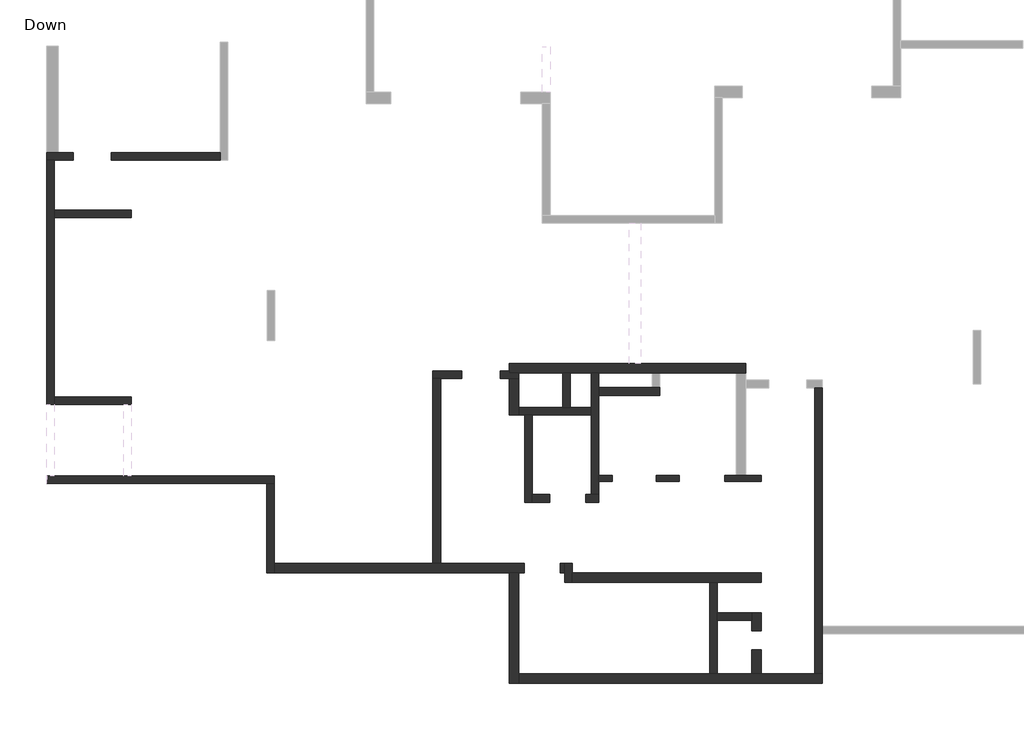
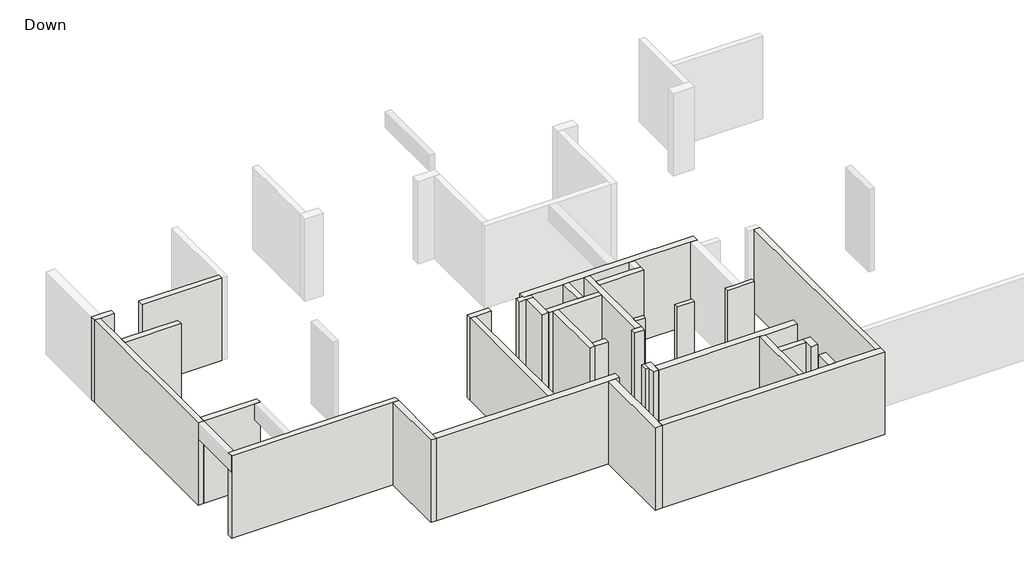
# One storey, part 1 of 2: 33 walls.
"""IFC4 building model written with IfcOpenShell, lengths in millimetres."""

from ifc_helpers import new_model, si_unit, origin, origin_with_axes, place, context, project, spatial, polyline, outline, extrude, faceted_brep, element, save

model = new_model("IFC4")

# Units and contexts
model_context = context("Model", 3, world=origin())
ifc_project = project(units=[si_unit("LENGTHUNIT", "METRE", prefix="MILLI")], contexts=[model_context])

# Site, building, storey
site = spatial("IfcSite", under=ifc_project)
building = spatial("IfcBuilding", under=site)
storey = spatial("IfcBuildingStorey", under=building, Name="Down", Elevation=0.0)

# Walls
placement = place(None, origin())
element("IfcWall", 1, ObjectType="15", at=placement, inside=storey, context=model_context, shape_type="Brep", body=[
    faceted_brep([(-5557.7212244, 6644.9881336, 0.0), (-5957.7212244, 6644.9881336, 0.0), (-6207.7212244, 6644.9881336, 0.0), (-6502.9843823, 6644.9881336, 0.0), (-6502.9843823, 6644.9881336, 3100.0), (-6207.7212244, 6644.9881336, 3100.0), (-5957.7212244, 6644.9881336, 3100.0), (-5557.7212244, 6644.9881336, 3100.0), (-5557.7212244, 6644.9881336, 2920.0), (-5557.7212244, 6494.9881336, 0.0), (-5557.7212244, 6494.9881336, 2920.0), (-5557.7212244, 6494.9881336, 3100.0), (-6502.9843823, 6494.9881336, 3100.0), (-6502.9843823, 6494.9881336, 2920.0), (-6502.9843823, 6494.9881336, 0.0), (-6502.9843823, 6644.4618178, 3100.0)], [[[0, 1, 2, 3, 4, 5, 6, 7, 8]], [[9, 10, 11, 12, 13, 14]], [[3, 2, 1, 0, 9, 14]], [[4, 3, 14, 13, 12, 15]], [[7, 6, 5, 4, 15, 12, 11]], [[0, 8, 7, 11, 10, 9]]]),
])
element("IfcWall", 2, ObjectType="15", at=placement, inside=storey, context=model_context, shape_type="Brep", body=[
    faceted_brep([(-7696.6685928, 6644.4618178, 0.0), (-8294.5633296, 6644.4618178, 0.0), (-8294.5633296, 6644.4618178, 2920.0), (-8294.5633296, 6644.4618178, 3100.0), (-7696.6685928, 6644.4618178, 3100.0), (-7696.6685928, 6644.4618178, 2920.0), (-7696.6685928, 6494.4618178, 0.0), (-7696.6685928, 6494.4618178, 2920.0), (-7696.6685928, 6494.4618178, 3100.0), (-8294.5633296, 6494.4618178, 3100.0), (-8294.5633296, 6494.4618178, 2920.0), (-8294.5633296, 6494.4618178, 0.0)], [[[0, 1, 2, 3, 4, 5]], [[6, 7, 8, 9, 10, 11]], [[1, 0, 6, 11]], [[3, 2, 1, 11, 10, 9]], [[4, 3, 9, 8]], [[0, 5, 4, 8, 7, 6]]]),
])
element("IfcWall", 3, ObjectType="15", at=placement, inside=storey, context=model_context, shape_type="Brep", body=[
    faceted_brep([(-9437.7212244, 6644.4618178, 0.0), (-9785.0896454, 6644.4618178, 0.0), (-9785.0896454, 6644.4618178, 3100.0), (-9437.7212244, 6644.4618178, 3100.0), (-9437.7212244, 6644.4618178, 2920.0), (-9437.7212244, 6494.4618178, 0.0), (-9437.7212244, 6494.4618178, 2920.0), (-9437.7212244, 6494.4618178, 3100.0), (-9785.0896454, 6494.4618178, 3100.0), (-9785.0896454, 6494.4618178, 2920.0), (-9785.0896454, 6494.4618178, 0.0)], [[[0, 1, 2, 3, 4]], [[5, 6, 7, 8, 9, 10]], [[1, 0, 5, 10]], [[3, 2, 8, 7]], [[0, 4, 3, 7, 6, 5]], [[2, 1, 10, 9, 8]]]),
])
element("IfcWall", 4, ObjectType="20", at=placement, inside=storey, context=model_context, shape_type="Brep", body=[
    faceted_brep([(-19660.8791191, 15061.303923, 0.0), (-22490.8791191, 15061.303923, 0.0), (-22490.8791191, 15061.303923, 2920.0), (-22490.8791191, 15061.303923, 3100.0), (-19660.8791191, 15061.303923, 3100.0), (-19660.8791191, 15061.303923, 2920.0), (-19660.8791191, 14861.303923, 0.0), (-19660.8791191, 14861.303923, 3100.0), (-22490.8791191, 14861.303923, 3100.0), (-22490.8791191, 14861.303923, 2920.0), (-22490.8791191, 14861.303923, 0.0)], [[[0, 1, 2, 3, 4, 5]], [[6, 7, 8, 9, 10]], [[1, 0, 6, 10]], [[3, 2, 1, 10, 9, 8]], [[4, 3, 8, 7]], [[0, 5, 4, 7, 6]]]),
])
element("IfcWall", 5, ObjectType="20", at=placement, inside=storey, context=model_context, shape_type="Brep", body=[
    faceted_brep([(-23484.0370138, 15061.303923, 0.0), (-23878.7738559, 15061.303923, 0.0), (-24178.7738559, 15061.303923, 0.0), (-24180.8791191, 15061.303923, 0.0), (-24180.8791191, 15061.303923, 3100.0), (-24178.7738559, 15061.303923, 3100.0), (-23878.7738559, 15061.303923, 3100.0), (-23484.0370138, 15061.303923, 3100.0), (-23484.0370138, 15061.303923, 2920.0), (-23484.0370138, 14861.303923, 0.0), (-23484.0370138, 14861.303923, 2920.0), (-23484.0370138, 14861.303923, 3100.0), (-23980.8791191, 14861.303923, 3100.0), (-24180.8791191, 14861.303923, 3100.0), (-24180.8791191, 14861.303923, 0.0), (-23980.8791191, 14861.303923, 0.0)], [[[0, 1, 2, 3, 4, 5, 6, 7, 8]], [[9, 10, 11, 12, 13, 14, 15]], [[3, 2, 1, 0, 9, 15, 14]], [[7, 6, 5, 4, 13, 12, 11]], [[0, 8, 7, 11, 10, 9]], [[4, 3, 14, 13]]]),
])
element("IfcWall", 6, ObjectType="20", at=placement, inside=storey, context=model_context, shape_type="Brep", body=[
    faceted_brep([(-24180.8791191, 14861.303923, 0.0), (-24180.8791191, 8497.0933967, 0.0), (-24180.8791191, 8497.0933967, 2500.0), (-24180.8791191, 8497.0933967, 3100.0), (-24180.8791191, 14861.303923, 3100.0), (-23980.8791191, 14861.303923, 0.0), (-23980.8791191, 14861.303923, 2920.0), (-23980.8791191, 14861.303923, 3100.0), (-23980.8791191, 13568.6723441, 3100.0), (-23980.8791191, 13368.6723441, 3100.0), (-23980.8791191, 8697.0933967, 3100.0), (-23980.8791191, 8497.0933967, 3100.0), (-23980.8791191, 8497.0933967, 2500.0), (-23980.8791191, 8497.0933967, 0.0), (-23980.8791191, 8697.0933967, 0.0), (-23980.8791191, 13368.6723441, 0.0), (-23980.8791191, 13568.6723441, 0.0)], [[[0, 1, 2, 3, 4]], [[5, 6, 7, 8, 9, 10, 11, 12, 13, 14, 15, 16]], [[1, 0, 5, 16, 15, 14, 13]], [[4, 3, 11, 10, 9, 8, 7]], [[0, 4, 7, 6, 5]], [[3, 2, 1, 13, 12, 11]]]),
])
element("IfcWall", 7, ObjectType="20", at=placement, inside=storey, context=model_context, shape_type="Brep", body=[
    faceted_brep([(-23980.8791191, 13368.6723441, 0.0), (-21970.3528033, 13368.6723441, 0.0), (-21970.3528033, 13368.6723441, 2920.0), (-21970.3528033, 13368.6723441, 3100.0), (-23980.8791191, 13368.6723441, 3100.0), (-23980.8791191, 13368.6723441, 2920.0), (-23980.8791191, 13568.6723441, 0.0), (-23980.8791191, 13568.6723441, 2920.0), (-23980.8791191, 13568.6723441, 3100.0), (-21970.3528033, 13568.6723441, 3100.0), (-21970.3528033, 13568.6723441, 2920.0), (-21970.3528033, 13568.6723441, 0.0)], [[[0, 1, 2, 3, 4, 5]], [[6, 7, 8, 9, 10, 11]], [[1, 0, 6, 11]], [[3, 2, 1, 11, 10, 9]], [[4, 3, 9, 8]], [[0, 5, 4, 8, 7, 6]]]),
])
element("IfcWall", 8, ObjectType="20", at=placement, inside=storey, context=model_context, shape_type="Brep", body=[
    faceted_brep([(-23980.8791191, 8497.0933967, 0.0), (-21970.3528033, 8497.0933967, 0.0), (-21970.3528033, 8497.0933967, 3100.0), (-22170.3528033, 8497.0933967, 3100.0), (-23980.8791191, 8497.0933967, 3100.0), (-23980.8791191, 8497.0933967, 2920.0), (-23980.8791191, 8697.0933967, 0.0), (-23980.8791191, 8697.0933967, 2920.0), (-23980.8791191, 8697.0933967, 3100.0), (-21970.3528033, 8697.0933967, 3100.0), (-21970.3528033, 8697.0933967, 2920.0), (-21970.3528033, 8697.0933967, 0.0)], [[[0, 1, 2, 3, 4, 5]], [[6, 7, 8, 9, 10, 11]], [[1, 0, 6, 11]], [[2, 1, 11, 10, 9]], [[4, 3, 2, 9, 8]], [[0, 5, 4, 8, 7, 6]]]),
])
element("IfcWall", 9, ObjectType="20", at=placement, inside=storey, context=model_context, shape_type="Brep", body=[
    faceted_brep([(-24178.7738559, 6438.1460283, 0.0), (-18441.9317507, 6438.1460283, 0.0), (-18241.9317507, 6438.1460283, 0.0), (-18241.9317507, 6438.1460283, 3100.0), (-18441.9317507, 6438.1460283, 3100.0), (-24178.7738559, 6438.1460283, 3100.0), (-24178.7738559, 6638.1460283, 0.0), (-24178.7738559, 6638.1460283, 3100.0), (-23980.8791191, 6638.1460283, 3100.0), (-22170.3528033, 6638.1460283, 3100.0), (-21970.3528033, 6638.1460283, 3100.0), (-18241.9317507, 6638.1460283, 3100.0), (-18241.9317507, 6638.1460283, 2920.0), (-18241.9317507, 6638.1460283, 0.0)], [[[0, 1, 2, 3, 4, 5]], [[6, 7, 8, 9, 10, 11, 12, 13]], [[2, 1, 0, 6, 13]], [[5, 4, 3, 11, 10, 9, 8, 7]], [[0, 5, 7, 6]], [[3, 2, 13, 12, 11]]]),
])
element("IfcWall", 10, ObjectType="20", at=placement, inside=storey, context=model_context, shape_type="Brep", body=[
    faceted_brep([(-18441.9317507, 6438.1460283, 0.0), (-18441.9317507, 4107.6197125, 0.0), (-18441.9317507, 4107.6197125, 3100.0), (-18441.9317507, 6438.1460283, 3100.0), (-18241.9317507, 6438.1460283, 0.0), (-18241.9317507, 6438.1460283, 3100.0), (-18241.9317507, 4357.6197125, 3100.0), (-18241.9317507, 4107.6197125, 3100.0), (-18241.9317507, 4107.6197125, 0.0), (-18241.9317507, 4357.6197125, 0.0)], [[[0, 1, 2, 3]], [[4, 5, 6, 7, 8, 9]], [[1, 0, 4, 9, 8]], [[3, 2, 7, 6, 5]], [[0, 3, 5, 4]], [[2, 1, 8, 7]]]),
])
element("IfcWall", 11, ObjectType="20", at=placement, inside=storey, context=model_context, shape_type="SweptSolid", body=[
    extrude(outline(polyline([(-6700.8791191, 3063.4091862), (-5809.8264875, 3063.4091862), (-5809.8264875, 2863.4091862), (-6700.8791191, 2863.4091862), (-6700.8791191, 3063.4091862)])), origin_with_axes(), (0.0, 0.0, 1.0), 3100.0),
])
element("IfcWall", 12, ObjectType="20", at=placement, inside=storey, context=model_context, shape_type="Brep", body=[
    faceted_brep([(-6700.8791191, 1473.4091862, 0.0), (-6700.8791191, 2863.4091862, 0.0), (-6700.8791191, 3063.4091862, 0.0), (-6700.8791191, 3859.1986599, 0.0), (-6700.8791191, 3859.1986599, 3100.0), (-6700.8791191, 3063.4091862, 3100.0), (-6700.8791191, 2863.4091862, 3100.0), (-6700.8791191, 1473.4091862, 3100.0), (-6900.8791191, 1473.4091862, 0.0), (-6900.8791191, 1473.4091862, 3100.0), (-6900.8791191, 3859.1986599, 3100.0), (-6900.8791191, 3859.1986599, 0.0)], [[[0, 1, 2, 3, 4, 5, 6, 7]], [[8, 9, 10, 11]], [[3, 2, 1, 0, 8, 11]], [[7, 6, 5, 4, 10, 9]], [[4, 3, 11, 10]], [[0, 7, 9, 8]]]),
])
element("IfcWall", 13, ObjectType="20", at=placement, inside=storey, context=model_context, shape_type="Brep", body=[
    faceted_brep([(-10481.9317507, 3859.1986599, 0.0), (-10481.9317507, 4109.1986599, 0.0), (-10481.9317507, 4358.1460283, 0.0), (-10481.9317507, 4358.1460283, 2920.0), (-10481.9317507, 4358.1460283, 3100.0), (-10481.9317507, 4109.1986599, 3100.0), (-10481.9317507, 3859.1986599, 3100.0), (-10681.9317507, 3859.1986599, 0.0), (-10681.9317507, 3859.1986599, 2920.0), (-10681.9317507, 3859.1986599, 3100.0), (-10681.9317507, 4108.1460283, 3100.0), (-10681.9317507, 4358.1460283, 3100.0), (-10681.9317507, 4358.1460283, 0.0), (-10681.9317507, 4108.1460283, 0.0)], [[[0, 1, 2, 3, 4, 5, 6]], [[7, 8, 9, 10, 11, 12, 13]], [[2, 1, 0, 7, 13, 12]], [[6, 5, 4, 11, 10, 9]], [[0, 6, 9, 8, 7]], [[4, 3, 2, 12, 11]]]),
])
element("IfcWall", 14, ObjectType="20", at=placement, inside=storey, context=model_context, shape_type="Brep", body=[
    faceted_brep([(-3966.142277, 1473.4091862, 0.0), (-3966.142277, 2516.0407652, 0.0), (-3966.142277, 2716.0407652, 0.0), (-3966.142277, 8930.7776073, 0.0), (-3966.142277, 8930.7776073, 3100.0), (-3966.142277, 2716.0407652, 3100.0), (-3966.142277, 2516.0407652, 3100.0), (-3966.142277, 1473.4091862, 3100.0), (-4166.142277, 1473.4091862, 0.0), (-4166.142277, 1473.4091862, 2920.0), (-4166.142277, 1473.4091862, 3100.0), (-4166.142277, 8930.7776073, 3100.0), (-4166.142277, 8930.7776073, 2920.0), (-4166.142277, 8930.7776073, 0.0)], [[[0, 1, 2, 3, 4, 5, 6, 7]], [[8, 9, 10, 11, 12, 13]], [[3, 2, 1, 0, 8, 13]], [[7, 6, 5, 4, 11, 10]], [[4, 3, 13, 12, 11]], [[0, 7, 10, 9, 8]]]),
])
element("IfcWall", 15, ObjectType="20", at=placement, inside=storey, context=model_context, shape_type="Brep", body=[
    faceted_brep([(-9785.0896454, 6147.6197125, 0.0), (-9785.0896454, 6494.4618178, 0.0), (-9785.0896454, 6644.4618178, 0.0), (-9785.0896454, 8732.8828704, 0.0), (-9785.0896454, 8932.8828704, 0.0), (-9785.0896454, 9312.3565546, 0.0), (-9785.0896454, 9312.3565546, 3100.0), (-9785.0896454, 8932.8828704, 3100.0), (-9785.0896454, 8732.8828704, 3100.0), (-9785.0896454, 6644.4618178, 3100.0), (-9785.0896454, 6494.4618178, 3100.0), (-9785.0896454, 6147.6197125, 3100.0), (-9985.0896454, 6147.6197125, 0.0), (-9985.0896454, 6147.6197125, 2920.0), (-9985.0896454, 6147.6197125, 3100.0), (-9985.0896454, 8219.1986599, 3100.0), (-9985.0896454, 8419.1986599, 3100.0), (-9985.0896454, 9312.3565546, 3100.0), (-9985.0896454, 9312.3565546, 0.0), (-9985.0896454, 8419.1986599, 0.0), (-9985.0896454, 8219.1986599, 0.0)], [[[0, 1, 2, 3, 4, 5, 6, 7, 8, 9, 10, 11]], [[12, 13, 14, 15, 16, 17, 18, 19, 20]], [[5, 4, 3, 2, 1, 0, 12, 20, 19, 18]], [[11, 10, 9, 8, 7, 6, 17, 16, 15, 14]], [[6, 5, 18, 17]], [[0, 11, 14, 13, 12]]]),
])
element("IfcWall", 16, ObjectType="20", at=placement, inside=storey, context=model_context, shape_type="SweptSolid", body=[
    extrude(outline(polyline([(-10728.2475402, 8419.1986599), (-10728.2475402, 9312.3565546), (-10528.2475402, 9312.3565546), (-10528.2475402, 8419.1986599), (-10728.2475402, 8419.1986599)])), origin_with_axes(), (0.0, 0.0, 1.0), 3100.0),
])
element("IfcWall", 17, ObjectType="20", at=placement, inside=storey, context=model_context, shape_type="Brep", body=[
    faceted_brep([(-9785.0896454, 8732.8828704, 0.0), (-8195.6159612, 8732.8828704, 0.0), (-8195.6159612, 8732.8828704, 3100.0), (-9785.0896454, 8732.8828704, 3100.0), (-9785.0896454, 8932.8828704, 0.0), (-9785.0896454, 8932.8828704, 3100.0), (-8395.6159612, 8932.8828704, 3100.0), (-8195.6159612, 8932.8828704, 3100.0), (-8195.6159612, 8932.8828704, 0.0), (-8395.6159612, 8932.8828704, 0.0)], [[[0, 1, 2, 3]], [[4, 5, 6, 7, 8, 9]], [[1, 0, 4, 9, 8]], [[3, 2, 7, 6, 5]], [[0, 3, 5, 4]], [[2, 1, 8, 7]]]),
])
element("IfcWall", 18, ObjectType="20", at=placement, inside=storey, context=model_context, shape_type="Brep", body=[
    faceted_brep([(-11874.0370138, 8219.1986599, 0.0), (-11726.142277, 8219.1986599, 0.0), (-11526.142277, 8219.1986599, 0.0), (-9985.0896454, 8219.1986599, 0.0), (-9985.0896454, 8219.1986599, 2920.0), (-9985.0896454, 8219.1986599, 3100.0), (-11526.142277, 8219.1986599, 3100.0), (-11726.142277, 8219.1986599, 3100.0), (-11874.0370138, 8219.1986599, 3100.0), (-11874.0370138, 8419.1986599, 0.0), (-11874.0370138, 8419.1986599, 3100.0), (-10728.2475402, 8419.1986599, 3100.0), (-10528.2475402, 8419.1986599, 3100.0), (-9985.0896454, 8419.1986599, 3100.0), (-9985.0896454, 8419.1986599, 0.0), (-10528.2475402, 8419.1986599, 0.0), (-10728.2475402, 8419.1986599, 0.0)], [[[0, 1, 2, 3, 4, 5, 6, 7, 8]], [[9, 10, 11, 12, 13, 14, 15, 16]], [[3, 2, 1, 0, 9, 16, 15, 14]], [[8, 7, 6, 5, 13, 12, 11, 10]], [[0, 8, 10, 9]], [[5, 4, 3, 14, 13]]]),
])
element("IfcWall", 19, ObjectType="20", at=placement, inside=storey, context=model_context, shape_type="Brep", body=[
    faceted_brep([(-11726.142277, 8219.1986599, 0.0), (-11726.142277, 5947.6197125, 0.0), (-11726.142277, 5947.6197125, 2920.0), (-11726.142277, 5947.6197125, 3100.0), (-11726.142277, 8219.1986599, 3100.0), (-11726.142277, 8219.1986599, 2920.0), (-11526.142277, 8219.1986599, 0.0), (-11526.142277, 8219.1986599, 2920.0), (-11526.142277, 8219.1986599, 3100.0), (-11526.142277, 6147.6197125, 3100.0), (-11526.142277, 5947.6197125, 3100.0), (-11526.142277, 5947.6197125, 0.0), (-11526.142277, 6147.6197125, 0.0)], [[[0, 1, 2, 3, 4, 5]], [[6, 7, 8, 9, 10, 11, 12]], [[1, 0, 6, 12, 11]], [[4, 3, 10, 9, 8]], [[0, 5, 4, 8, 7, 6]], [[3, 2, 1, 11, 10]]]),
])
element("IfcWall", 20, ObjectType="20", at=placement, inside=storey, context=model_context, shape_type="Brep", body=[
    faceted_brep([(-11526.142277, 5947.6197125, 0.0), (-11069.3001717, 5947.6197125, 0.0), (-11069.3001717, 5947.6197125, 2920.0), (-11069.3001717, 5947.6197125, 3100.0), (-11526.142277, 5947.6197125, 3100.0), (-11526.142277, 6147.6197125, 0.0), (-11526.142277, 6147.6197125, 2920.0), (-11526.142277, 6147.6197125, 3100.0), (-11069.3001717, 6147.6197125, 3100.0), (-11069.3001717, 6147.6197125, 2920.0), (-11069.3001717, 6147.6197125, 0.0)], [[[0, 1, 2, 3, 4]], [[5, 6, 7, 8, 9, 10]], [[1, 0, 5, 10]], [[3, 2, 1, 10, 9, 8]], [[4, 3, 8, 7]], [[0, 4, 7, 6, 5]]]),
])
element("IfcWall", 21, ObjectType="20", at=placement, inside=storey, context=model_context, shape_type="Brep", body=[
    faceted_brep([(-10124.0370138, 5947.6197125, 0.0), (-9785.0896454, 5947.6197125, 0.0), (-9785.0896454, 5947.6197125, 2920.0), (-9785.0896454, 5947.6197125, 3100.0), (-10124.0370138, 5947.6197125, 3100.0), (-10124.0370138, 5947.6197125, 2920.0), (-10124.0370138, 6147.6197125, 0.0), (-10124.0370138, 6147.6197125, 2920.0), (-10124.0370138, 6147.6197125, 3100.0), (-9985.0896454, 6147.6197125, 3100.0), (-9785.0896454, 6147.6197125, 3100.0), (-9785.0896454, 6147.6197125, 0.0), (-9985.0896454, 6147.6197125, 0.0)], [[[0, 1, 2, 3, 4, 5]], [[6, 7, 8, 9, 10, 11, 12]], [[1, 0, 6, 12, 11]], [[4, 3, 10, 9, 8]], [[0, 5, 4, 8, 7, 6]], [[3, 2, 1, 11, 10]]]),
])
element("IfcWall", 22, ObjectType="20", at=placement, inside=storey, context=model_context, shape_type="Brep", body=[
    faceted_brep([(-12364.0370138, 9370.9220034, 0.0), (-12364.0370138, 9370.9220034, 2920.0), (-12364.0370138, 9370.9220034, 3100.0), (-12124.0370138, 9370.9220034, 3100.0), (-12124.0370138, 9370.9220034, 2920.0), (-12124.0370138, 9370.9220034, 0.0), (-12364.0370138, 9170.9220034, 0.0), (-12124.0370138, 9170.9220034, 0.0), (-11874.0370138, 9170.9220034, 0.0), (-11874.0370138, 9170.9220034, 3100.0), (-12124.0370138, 9170.9220034, 3100.0), (-12364.0370138, 9170.9220034, 3100.0), (-12364.0370138, 9170.9220034, 2920.0), (-12124.0370138, 9312.3565546, 0.0), (-11874.0370138, 9312.3565546, 0.0), (-11874.0370138, 9312.3565546, 3100.0), (-12124.0370138, 9312.3565546, 3100.0)], [[[0, 1, 2, 3, 4, 5]], [[6, 7, 8, 9, 10, 11, 12]], [[8, 7, 6, 0, 5, 13, 14]], [[2, 1, 0, 6, 12, 11]], [[11, 10, 9, 15, 16, 3, 2]], [[9, 8, 14, 15]], [[13, 16, 15, 14]], [[16, 13, 5, 4, 3]]]),
])
element("IfcWall", 23, ObjectType="20", at=placement, inside=storey, context=model_context, shape_type="Brep", body=[
    faceted_brep([(-13360.7601979, 9370.9220034, 0.0), (-14113.5106981, 9370.9220034, 0.0), (-14113.5106981, 9370.9220034, 2920.0), (-14113.5106981, 9370.9220034, 3100.0), (-13360.7601979, 9370.9220034, 3100.0), (-13360.7601979, 9370.9220034, 2920.0), (-13360.7601979, 9170.9220034, 0.0), (-13360.7601979, 9170.9220034, 2920.0), (-13360.7601979, 9170.9220034, 3100.0), (-13913.5106981, 9170.9220034, 3100.0), (-14113.5106981, 9170.9220034, 3100.0), (-14113.5106981, 9170.9220034, 0.0), (-13913.5106981, 9170.9220034, 0.0)], [[[0, 1, 2, 3, 4, 5]], [[6, 7, 8, 9, 10, 11, 12]], [[1, 0, 6, 12, 11]], [[4, 3, 10, 9, 8]], [[0, 5, 4, 8, 7, 6]], [[3, 2, 1, 11, 10]]]),
])
element("IfcWall", 24, ObjectType="20", at=placement, inside=storey, context=model_context, shape_type="Brep", body=[
    faceted_brep([(-14113.5106981, 9170.9220034, 0.0), (-14113.5106981, 4357.6197125, 0.0), (-14113.5106981, 4357.6197125, 2920.0), (-14113.5106981, 4357.6197125, 3100.0), (-14113.5106981, 9170.9220034, 3100.0), (-13913.5106981, 9170.9220034, 0.0), (-13913.5106981, 9170.9220034, 2920.0), (-13913.5106981, 9170.9220034, 3100.0), (-13913.5106981, 4357.6197125, 3100.0), (-13913.5106981, 4357.6197125, 2920.0), (-13913.5106981, 4357.6197125, 0.0)], [[[0, 1, 2, 3, 4]], [[5, 6, 7, 8, 9, 10]], [[1, 0, 5, 10]], [[4, 3, 8, 7]], [[0, 4, 7, 6, 5]], [[3, 2, 1, 10, 9, 8]]]),
])
element("IfcWall", 25, ObjectType="25", at=placement, inside=storey, context=model_context, shape_type="Brep", body=[
    faceted_brep([(-18241.9317507, 4107.6197125, 0.0), (-12125.6159612, 4107.6197125, 0.0), (-11875.6159612, 4107.6197125, 0.0), (-11736.6685928, 4107.6197125, 0.0), (-11736.6685928, 4107.6197125, 2920.0), (-11736.6685928, 4107.6197125, 3100.0), (-11875.6159612, 4107.6197125, 3100.0), (-12125.6159612, 4107.6197125, 3100.0), (-18241.9317507, 4107.6197125, 3100.0), (-18241.9317507, 4357.6197125, 0.0), (-18241.9317507, 4357.6197125, 2920.0), (-18241.9317507, 4357.6197125, 3100.0), (-14113.5106981, 4357.6197125, 3100.0), (-13913.5106981, 4357.6197125, 3100.0), (-11736.6685928, 4357.6197125, 3100.0), (-11736.6685928, 4357.6197125, 2920.0), (-11736.6685928, 4357.6197125, 0.0), (-13913.5106981, 4357.6197125, 0.0), (-14113.5106981, 4357.6197125, 0.0)], [[[0, 1, 2, 3, 4, 5, 6, 7, 8]], [[9, 10, 11, 12, 13, 14, 15, 16, 17, 18]], [[3, 2, 1, 0, 9, 18, 17, 16]], [[5, 4, 3, 16, 15, 14]], [[8, 7, 6, 5, 14, 13, 12, 11]], [[0, 8, 11, 10, 9]]]),
])
element("IfcWall", 26, ObjectType="25", at=placement, inside=storey, context=model_context, shape_type="Brep", body=[
    faceted_brep([(-12125.6159612, 4107.6197125, 0.0), (-12125.6159612, 1223.4091862, 0.0), (-12125.6159612, 1223.4091862, 3100.0), (-12125.6159612, 4107.6197125, 3100.0), (-11875.6159612, 4107.6197125, 0.0), (-11875.6159612, 4107.6197125, 2920.0), (-11875.6159612, 4107.6197125, 3100.0), (-11875.6159612, 1473.4091862, 3100.0), (-11875.6159612, 1223.4091862, 3100.0), (-11875.6159612, 1223.4091862, 0.0), (-11875.6159612, 1473.4091862, 0.0)], [[[0, 1, 2, 3]], [[4, 5, 6, 7, 8, 9, 10]], [[1, 0, 4, 10, 9]], [[3, 2, 8, 7, 6]], [[0, 3, 6, 5, 4]], [[2, 1, 9, 8]]]),
])
element("IfcWall", 27, ObjectType="25", at=placement, inside=storey, context=model_context, shape_type="Brep", body=[
    faceted_brep([(-11875.6159612, 1223.4091862, 0.0), (-3966.142277, 1223.4091862, 0.0), (-3966.142277, 1223.4091862, 3100.0), (-11875.6159612, 1223.4091862, 3100.0), (-11875.6159612, 1473.4091862, 0.0), (-11875.6159612, 1473.4091862, 2920.0), (-11875.6159612, 1473.4091862, 3100.0), (-10462.9843823, 1473.4091862, 3100.0), (-6900.8791191, 1473.4091862, 3100.0), (-6700.8791191, 1473.4091862, 3100.0), (-5809.8264875, 1473.4091862, 3100.0), (-5559.8264875, 1473.4091862, 3100.0), (-4166.142277, 1473.4091862, 3100.0), (-3966.142277, 1473.4091862, 3100.0), (-3966.142277, 1473.4091862, 0.0), (-4166.142277, 1473.4091862, 0.0), (-5559.8264875, 1473.4091862, 0.0), (-5809.8264875, 1473.4091862, 0.0), (-6700.8791191, 1473.4091862, 0.0), (-6900.8791191, 1473.4091862, 0.0)], [[[0, 1, 2, 3]], [[4, 5, 6, 7, 8, 9, 10, 11, 12, 13, 14, 15, 16, 17, 18, 19]], [[1, 0, 4, 19, 18, 17, 16, 15, 14]], [[3, 2, 13, 12, 11, 10, 9, 8, 7, 6]], [[0, 3, 6, 5, 4]], [[2, 1, 14, 13]]]),
])
element("IfcWall", 28, ObjectType="25", at=placement, inside=storey, context=model_context, shape_type="Brep", body=[
    faceted_brep([(-5559.8264875, 1473.4091862, 0.0), (-5559.8264875, 2094.9881336, 0.0), (-5559.8264875, 2094.9881336, 3100.0), (-5559.8264875, 1473.4091862, 3100.0), (-5559.8264875, 1473.4091862, 2920.0), (-5809.8264875, 1473.4091862, 0.0), (-5809.8264875, 1473.4091862, 3100.0), (-5809.8264875, 2094.9881336, 3100.0), (-5809.8264875, 2094.9881336, 0.0)], [[[0, 1, 2, 3, 4]], [[5, 6, 7, 8]], [[1, 0, 5, 8]], [[2, 1, 8, 7]], [[3, 2, 7, 6]], [[0, 4, 3, 6, 5]]]),
])
element("IfcWall", 29, ObjectType="25", at=placement, inside=storey, context=model_context, shape_type="Brep", body=[
    faceted_brep([(-5559.8264875, 2591.8302388, 0.0), (-5559.8264875, 3063.4091862, 0.0), (-5559.8264875, 3063.4091862, 3100.0), (-5559.8264875, 2591.8302388, 3100.0), (-5809.8264875, 2591.8302388, 0.0), (-5809.8264875, 2591.8302388, 3100.0), (-5809.8264875, 2863.4091862, 3100.0), (-5809.8264875, 3063.4091862, 3100.0), (-5809.8264875, 3063.4091862, 0.0), (-5809.8264875, 2863.4091862, 0.0)], [[[0, 1, 2, 3]], [[4, 5, 6, 7, 8, 9]], [[1, 0, 4, 9, 8]], [[3, 2, 7, 6, 5]], [[0, 3, 5, 4]], [[2, 1, 8, 7]]]),
])
element("IfcWall", 30, ObjectType="25", at=placement, inside=storey, context=model_context, shape_type="Brep", body=[
    faceted_brep([(-5559.8264875, 4109.1986599, 0.0), (-10481.9317507, 4109.1986599, 0.0), (-10481.9317507, 4109.1986599, 2920.0), (-10481.9317507, 4109.1986599, 3100.0), (-5559.8264875, 4109.1986599, 3100.0), (-5559.8264875, 4109.1986599, 2920.0), (-5559.8264875, 3859.1986599, 0.0), (-5559.8264875, 3859.1986599, 3100.0), (-6700.8791191, 3859.1986599, 3100.0), (-6900.8791191, 3859.1986599, 3100.0), (-10462.9843823, 3859.1986599, 3100.0), (-10481.9317507, 3859.1986599, 3100.0), (-10481.9317507, 3859.1986599, 0.0), (-6900.8791191, 3859.1986599, 0.0), (-6700.8791191, 3859.1986599, 0.0)], [[[0, 1, 2, 3, 4, 5]], [[6, 7, 8, 9, 10, 11, 12, 13, 14]], [[1, 0, 6, 14, 13, 12]], [[4, 3, 11, 10, 9, 8, 7]], [[0, 5, 4, 7, 6]], [[3, 2, 1, 12, 11]]]),
])
element("IfcWall", 31, ObjectType="25", at=placement, inside=storey, context=model_context, shape_type="Brep", body=[
    faceted_brep([(-10681.9317507, 4358.1460283, 0.0), (-10791.4054349, 4358.1460283, 0.0), (-10791.4054349, 4358.1460283, 2920.0), (-10791.4054349, 4358.1460283, 3100.0), (-10681.9317507, 4358.1460283, 3100.0), (-10681.9317507, 4108.1460283, 0.0), (-10681.9317507, 4108.1460283, 2920.0), (-10681.9317507, 4108.1460283, 3100.0), (-10791.4054349, 4108.1460283, 3100.0), (-10791.4054349, 4108.1460283, 2920.0), (-10791.4054349, 4108.1460283, 0.0)], [[[0, 1, 2, 3, 4]], [[5, 6, 7, 8, 9, 10]], [[1, 0, 5, 10]], [[3, 2, 1, 10, 9, 8]], [[4, 3, 8, 7]], [[0, 4, 7, 6, 5]]]),
])
element("IfcWall", 32, ObjectType="25", at=placement, inside=storey, context=model_context, shape_type="Brep", body=[
    faceted_brep([(-5957.7212244, 9562.3565546, 0.0), (-12124.0370138, 9562.3565546, 0.0), (-12124.0370138, 9562.3565546, 2920.0), (-12124.0370138, 9562.3565546, 3100.0), (-8991.4054349, 9562.3565546, 3100.0), (-8691.4054349, 9562.3565546, 3100.0), (-5957.7212244, 9562.3565546, 3100.0), (-5957.7212244, 9562.3565546, 2920.0), (-5957.7212244, 9312.3565546, 0.0), (-5957.7212244, 9312.3565546, 3100.0), (-6207.7212244, 9312.3565546, 3100.0), (-8195.6159612, 9312.3565546, 3100.0), (-8395.6159612, 9312.3565546, 3100.0), (-9785.0896454, 9312.3565546, 3100.0), (-9985.0896454, 9312.3565546, 3100.0), (-10528.2475402, 9312.3565546, 3100.0), (-10728.2475402, 9312.3565546, 3100.0), (-11874.0370138, 9312.3565546, 3100.0), (-12124.0370138, 9312.3565546, 3100.0), (-12124.0370138, 9312.3565546, 0.0), (-11874.0370138, 9312.3565546, 0.0), (-10728.2475402, 9312.3565546, 0.0), (-10528.2475402, 9312.3565546, 0.0), (-9985.0896454, 9312.3565546, 0.0), (-9785.0896454, 9312.3565546, 0.0), (-8395.6159612, 9312.3565546, 0.0), (-8195.6159612, 9312.3565546, 0.0), (-6207.7212244, 9312.3565546, 0.0), (-12124.0370138, 9370.9220034, 0.0), (-12124.0370138, 9370.9220034, 3100.0)], [[[0, 1, 2, 3, 4, 5, 6, 7]], [[8, 9, 10, 11, 12, 13, 14, 15, 16, 17, 18, 19, 20, 21, 22, 23, 24, 25, 26, 27]], [[1, 0, 8, 27, 26, 25, 24, 23, 22, 21, 20, 19, 28]], [[3, 2, 1, 28, 19, 18, 29]], [[6, 5, 4, 3, 29, 18, 17, 16, 15, 14, 13, 12, 11, 10, 9]], [[0, 7, 6, 9, 8]]]),
])
element("IfcWall", 33, ObjectType="25", at=placement, inside=storey, context=model_context, shape_type="Brep", body=[
    faceted_brep([(-12124.0370138, 9170.9220034, 0.0), (-12124.0370138, 8219.1986599, 0.0), (-12124.0370138, 8219.1986599, 2920.0), (-12124.0370138, 8219.1986599, 3100.0), (-12124.0370138, 9170.9220034, 3100.0), (-12124.0370138, 9170.9220034, 2920.0), (-11874.0370138, 9170.9220034, 0.0), (-11874.0370138, 9170.9220034, 3100.0), (-11874.0370138, 8419.1986599, 3100.0), (-11874.0370138, 8219.1986599, 3100.0), (-11874.0370138, 8219.1986599, 0.0), (-11874.0370138, 8419.1986599, 0.0)], [[[0, 1, 2, 3, 4, 5]], [[6, 7, 8, 9, 10, 11]], [[1, 0, 6, 11, 10]], [[4, 3, 9, 8, 7]], [[3, 2, 1, 10, 9]], [[0, 5, 4, 7, 6]]]),
])

save(model, "model.ifc")

# Revit data of these elements
# Project information
#   Project Issue Date = "Issue Date"
#   Project Status = "Project Status"
#   Client Name = "לקוח"
#   Project Address = "Enter address here"
#   Project Name = "Project 037"
#   Project Number = "מספר פרויקט"
# Type "15"
#   Layers, outside or top first: 15 cm "Concrete" (function 1)
# Type "20"
#   Layers, outside or top first: 20 cm "Concrete" (function 1)
# Type "25"
#   Layers, outside or top first: 25 cm "Concrete" (function 1)
# Element 1 (IfcWall, "15")
#   Comments = ""
#   Mark = "W61"
#   SOFiSTiK_EdgeZones = "W69"
#   SOFiSTiK_AMG_Comments = ""
#   Top Offset = 0 cm
#   Base Offset = 0 cm
#   wall height = 310 cm
#   SOFiSTiK_AMG_Scheduled = yes
#   SOFiSTiK_AMG_Adjusted = yes
#   Phase Created = New Construction
#   Base Constraint = Down
#   Top Constraint = Typical Floor
#   Materials on its faces: "Concrete"
# Element 2 (IfcWall, "15")
#   Comments = ""
#   Mark = "W62"
#   SOFiSTiK_EdgeZones = "W70"
#   SOFiSTiK_AMG_Comments = ""
#   Top Offset = 0 cm
#   Base Offset = 0 cm
#   wall height = 310 cm
#   SOFiSTiK_AMG_Scheduled = yes
#   SOFiSTiK_AMG_Adjusted = yes
#   Phase Created = New Construction
#   Base Constraint = Down
#   Top Constraint = Typical Floor
#   Materials on its faces: "Concrete"
# Element 3 (IfcWall, "15")
#   Comments = ""
#   Mark = "W63"
#   SOFiSTiK_EdgeZones = "W71"
#   SOFiSTiK_AMG_Comments = ""
#   Top Offset = 0 cm
#   Base Offset = 0 cm
#   wall height = 310 cm
#   SOFiSTiK_AMG_Scheduled = yes
#   SOFiSTiK_AMG_Adjusted = yes
#   Phase Created = New Construction
#   Base Constraint = Down
#   Top Constraint = Typical Floor
#   Materials on its faces: "Concrete"
# Element 4 (IfcWall, "20")
#   Comments = ""
#   Mark = "W3"
#   SOFiSTiK_EdgeZones = "W3"
#   SOFiSTiK_AMG_Comments = ""
#   Top Offset = 0 cm
#   Base Offset = 0 cm
#   wall height = 310 cm
#   SOFiSTiK_AMG_Scheduled = yes
#   SOFiSTiK_AMG_Adjusted = yes
#   Phase Created = New Construction
#   Base Constraint = Down
#   Top Constraint = Typical Floor
#   Materials on its faces: "Concrete"
# Element 5 (IfcWall, "20")
#   Comments = ""
#   Mark = "W4"
#   SOFiSTiK_EdgeZones = "W4"
#   SOFiSTiK_AMG_Comments = ""
#   Top Offset = 0 cm
#   Base Offset = 0 cm
#   wall height = 310 cm
#   SOFiSTiK_AMG_Scheduled = yes
#   SOFiSTiK_AMG_Adjusted = yes
#   Phase Created = New Construction
#   Base Constraint = Down
#   Top Constraint = Typical Floor
#   Materials on its faces: "Concrete"
# Element 6 (IfcWall, "20")
#   Comments = ""
#   Mark = "W5"
#   SOFiSTiK_EdgeZones = "W5"
#   SOFiSTiK_AMG_Comments = ""
#   Top Offset = 0 cm
#   Base Offset = 0 cm
#   wall height = 310 cm
#   SOFiSTiK_AMG_Scheduled = yes
#   SOFiSTiK_AMG_Adjusted = yes
#   Phase Created = New Construction
#   Base Constraint = Down
#   Top Constraint = Typical Floor
#   Materials on its faces: "Concrete"
# Element 7 (IfcWall, "20")
#   Comments = ""
#   Mark = "W6"
#   SOFiSTiK_EdgeZones = "W6"
#   SOFiSTiK_AMG_Comments = ""
#   Top Offset = 0 cm
#   Base Offset = 0 cm
#   wall height = 310 cm
#   SOFiSTiK_AMG_Scheduled = yes
#   SOFiSTiK_AMG_Adjusted = yes
#   Phase Created = New Construction
#   Base Constraint = Down
#   Top Constraint = Typical Floor
#   Materials on its faces: "Concrete"
# Element 8 (IfcWall, "20")
#   Comments = ""
#   Mark = "W7"
#   SOFiSTiK_EdgeZones = "W7"
#   SOFiSTiK_AMG_Comments = ""
#   Top Offset = 0 cm
#   Base Offset = 0 cm
#   wall height = 310 cm
#   SOFiSTiK_AMG_Scheduled = yes
#   SOFiSTiK_AMG_Adjusted = yes
#   Phase Created = New Construction
#   Base Constraint = Down
#   Top Constraint = Typical Floor
#   Materials on its faces: "Concrete"
# Element 9 (IfcWall, "20")
#   Comments = ""
#   Mark = "W8"
#   SOFiSTiK_EdgeZones = "W8"
#   SOFiSTiK_AMG_Comments = ""
#   Top Offset = 0 cm
#   Base Offset = 0 cm
#   wall height = 310 cm
#   SOFiSTiK_AMG_Scheduled = yes
#   SOFiSTiK_AMG_Adjusted = yes
#   Phase Created = New Construction
#   Base Constraint = Down
#   Top Constraint = Typical Floor
#   Materials on its faces: "Concrete"
# Element 10 (IfcWall, "20")
#   Comments = ""
#   Mark = "W9"
#   SOFiSTiK_EdgeZones = "W9"
#   SOFiSTiK_AMG_Comments = ""
#   Top Offset = 0 cm
#   Base Offset = 0 cm
#   wall height = 310 cm
#   SOFiSTiK_AMG_Scheduled = yes
#   SOFiSTiK_AMG_Adjusted = yes
#   Phase Created = New Construction
#   Base Constraint = Down
#   Top Constraint = Typical Floor
#   Materials on its faces: "Concrete"
# Element 11 (IfcWall, "20")
#   Comments = ""
#   Mark = "W10"
#   SOFiSTiK_EdgeZones = "W10"
#   SOFiSTiK_AMG_Comments = ""
#   Top Offset = 0 cm
#   Base Offset = 0 cm
#   wall height = 310 cm
#   SOFiSTiK_AMG_Scheduled = yes
#   SOFiSTiK_AMG_Adjusted = yes
#   Phase Created = New Construction
#   Base Constraint = Down
#   Top Constraint = Typical Floor
#   Materials on its faces: "Concrete"
# Element 12 (IfcWall, "20")
#   Comments = ""
#   Mark = "W11"
#   SOFiSTiK_EdgeZones = "W12"
#   SOFiSTiK_AMG_Comments = ""
#   Top Offset = 0 cm
#   Base Offset = 0 cm
#   wall height = 310 cm
#   SOFiSTiK_AMG_Scheduled = yes
#   SOFiSTiK_AMG_Adjusted = yes
#   Phase Created = New Construction
#   Base Constraint = Down
#   Top Constraint = Typical Floor
#   Materials on its faces: "Concrete"
# Element 13 (IfcWall, "20")
#   Comments = ""
#   Mark = "W12"
#   SOFiSTiK_EdgeZones = "W13"
#   SOFiSTiK_AMG_Comments = ""
#   Top Offset = 0 cm
#   Base Offset = 0 cm
#   wall height = 310 cm
#   SOFiSTiK_AMG_Scheduled = yes
#   SOFiSTiK_AMG_Adjusted = yes
#   Phase Created = New Construction
#   Base Constraint = Down
#   Top Constraint = Typical Floor
#   Materials on its faces: "Concrete"
# Element 14 (IfcWall, "20")
#   Comments = ""
#   Mark = "W29"
#   SOFiSTiK_EdgeZones = "W34"
#   SOFiSTiK_AMG_Comments = ""
#   Top Offset = 0 cm
#   Base Offset = 0 cm
#   wall height = 310 cm
#   SOFiSTiK_AMG_Scheduled = yes
#   SOFiSTiK_AMG_Adjusted = yes
#   Phase Created = New Construction
#   Base Constraint = Down
#   Top Constraint = Typical Floor
#   Materials on its faces: "Concrete"
# Element 15 (IfcWall, "20")
#   Comments = ""
#   Mark = "W32"
#   SOFiSTiK_EdgeZones = "W37"
#   SOFiSTiK_AMG_Comments = ""
#   Top Offset = 0 cm
#   Base Offset = 0 cm
#   wall height = 310 cm
#   SOFiSTiK_AMG_Scheduled = yes
#   SOFiSTiK_AMG_Adjusted = yes
#   Phase Created = New Construction
#   Base Constraint = Down
#   Top Constraint = Typical Floor
#   Materials on its faces: "Concrete"
# Element 16 (IfcWall, "20")
#   Comments = ""
#   Mark = "W33"
#   SOFiSTiK_EdgeZones = "W38"
#   SOFiSTiK_AMG_Comments = ""
#   Top Offset = 0 cm
#   Base Offset = 0 cm
#   wall height = 310 cm
#   SOFiSTiK_AMG_Scheduled = yes
#   SOFiSTiK_AMG_Adjusted = yes
#   Phase Created = New Construction
#   Base Constraint = Down
#   Top Constraint = Typical Floor
#   Materials on its faces: "Concrete"
# Element 17 (IfcWall, "20")
#   Comments = ""
#   Mark = "W34"
#   SOFiSTiK_EdgeZones = "W39"
#   SOFiSTiK_AMG_Comments = ""
#   Top Offset = 0 cm
#   Base Offset = 0 cm
#   wall height = 310 cm
#   SOFiSTiK_AMG_Scheduled = yes
#   SOFiSTiK_AMG_Adjusted = yes
#   Phase Created = New Construction
#   Base Constraint = Down
#   Top Constraint = Typical Floor
#   Materials on its faces: "Concrete"
# Element 18 (IfcWall, "20")
#   Comments = ""
#   Mark = "W36"
#   SOFiSTiK_EdgeZones = "W41"
#   SOFiSTiK_AMG_Comments = ""
#   Top Offset = 0 cm
#   Base Offset = 0 cm
#   wall height = 310 cm
#   SOFiSTiK_AMG_Scheduled = yes
#   SOFiSTiK_AMG_Adjusted = yes
#   Phase Created = New Construction
#   Base Constraint = Down
#   Top Constraint = Typical Floor
#   Materials on its faces: "Concrete"
# Element 19 (IfcWall, "20")
#   Comments = ""
#   Mark = "W37"
#   SOFiSTiK_EdgeZones = "W42"
#   SOFiSTiK_AMG_Comments = ""
#   Top Offset = 0 cm
#   Base Offset = 0 cm
#   wall height = 310 cm
#   SOFiSTiK_AMG_Scheduled = yes
#   SOFiSTiK_AMG_Adjusted = yes
#   Phase Created = New Construction
#   Base Constraint = Down
#   Top Constraint = Typical Floor
#   Materials on its faces: "Concrete"
# Element 20 (IfcWall, "20")
#   Comments = ""
#   Mark = "W38"
#   SOFiSTiK_EdgeZones = "W43"
#   SOFiSTiK_AMG_Comments = ""
#   Top Offset = 0 cm
#   Base Offset = 0 cm
#   wall height = 310 cm
#   SOFiSTiK_AMG_Scheduled = yes
#   SOFiSTiK_AMG_Adjusted = yes
#   Phase Created = New Construction
#   Base Constraint = Down
#   Top Constraint = Typical Floor
#   Materials on its faces: "Concrete"
# Element 21 (IfcWall, "20")
#   Comments = ""
#   Mark = "W39"
#   SOFiSTiK_EdgeZones = "W44"
#   SOFiSTiK_AMG_Comments = ""
#   Top Offset = 0 cm
#   Base Offset = 0 cm
#   wall height = 310 cm
#   SOFiSTiK_AMG_Scheduled = yes
#   SOFiSTiK_AMG_Adjusted = yes
#   Phase Created = New Construction
#   Base Constraint = Down
#   Top Constraint = Typical Floor
#   Materials on its faces: "Concrete"
# Element 22 (IfcWall, "20")
#   Comments = ""
#   Mark = "W40"
#   SOFiSTiK_EdgeZones = "W46"
#   SOFiSTiK_AMG_Comments = ""
#   Top Offset = 0 cm
#   Base Offset = 0 cm
#   wall height = 310 cm
#   SOFiSTiK_AMG_Scheduled = yes
#   SOFiSTiK_AMG_Adjusted = yes
#   Phase Created = New Construction
#   Base Constraint = Down
#   Top Constraint = Typical Floor
#   Materials on its faces: "Concrete"
# Element 23 (IfcWall, "20")
#   Comments = ""
#   Mark = "W41"
#   SOFiSTiK_EdgeZones = "W47"
#   SOFiSTiK_AMG_Comments = ""
#   Top Offset = 0 cm
#   Base Offset = 0 cm
#   wall height = 310 cm
#   SOFiSTiK_AMG_Scheduled = yes
#   SOFiSTiK_AMG_Adjusted = yes
#   Phase Created = New Construction
#   Base Constraint = Down
#   Top Constraint = Typical Floor
#   Materials on its faces: "Concrete"
# Element 24 (IfcWall, "20")
#   Comments = ""
#   Mark = "W42"
#   SOFiSTiK_EdgeZones = "W48"
#   SOFiSTiK_AMG_Comments = ""
#   Top Offset = 0 cm
#   Base Offset = 0 cm
#   wall height = 310 cm
#   SOFiSTiK_AMG_Scheduled = yes
#   SOFiSTiK_AMG_Adjusted = yes
#   Phase Created = New Construction
#   Base Constraint = Down
#   Top Constraint = Typical Floor
#   Materials on its faces: "Concrete"
# Element 25 (IfcWall, "25")
#   Comments = ""
#   Mark = "W43"
#   SOFiSTiK_EdgeZones = "W49"
#   SOFiSTiK_AMG_Comments = ""
#   Top Offset = 0 cm
#   Base Offset = 0 cm
#   wall height = 310 cm
#   SOFiSTiK_AMG_Scheduled = yes
#   SOFiSTiK_AMG_Adjusted = yes
#   Phase Created = New Construction
#   Base Constraint = Down
#   Top Constraint = Typical Floor
#   Materials on its faces: "Concrete"
# Element 26 (IfcWall, "25")
#   Comments = ""
#   Mark = "W44"
#   SOFiSTiK_EdgeZones = "W50"
#   SOFiSTiK_AMG_Comments = ""
#   Top Offset = 0 cm
#   Base Offset = 0 cm
#   wall height = 310 cm
#   SOFiSTiK_AMG_Scheduled = yes
#   SOFiSTiK_AMG_Adjusted = yes
#   Phase Created = New Construction
#   Base Constraint = Down
#   Top Constraint = Typical Floor
#   Materials on its faces: "Concrete"
# Element 27 (IfcWall, "25")
#   Comments = ""
#   Mark = "W45"
#   SOFiSTiK_EdgeZones = "W51"
#   SOFiSTiK_AMG_Comments = ""
#   Top Offset = 0 cm
#   Base Offset = 0 cm
#   wall height = 310 cm
#   SOFiSTiK_AMG_Scheduled = yes
#   SOFiSTiK_AMG_Adjusted = yes
#   Phase Created = New Construction
#   Base Constraint = Down
#   Top Constraint = Typical Floor
#   Materials on its faces: "Concrete"
# Element 28 (IfcWall, "25")
#   Comments = ""
#   Mark = "W46"
#   SOFiSTiK_EdgeZones = "W52"
#   SOFiSTiK_AMG_Comments = ""
#   Top Offset = 0 cm
#   Base Offset = 0 cm
#   wall height = 310 cm
#   SOFiSTiK_AMG_Scheduled = yes
#   SOFiSTiK_AMG_Adjusted = yes
#   Phase Created = New Construction
#   Base Constraint = Down
#   Top Constraint = Typical Floor
#   Materials on its faces: "Concrete"
# Element 29 (IfcWall, "25")
#   Comments = ""
#   Mark = "W47"
#   SOFiSTiK_EdgeZones = "W53"
#   SOFiSTiK_AMG_Comments = ""
#   Top Offset = 0 cm
#   Base Offset = 0 cm
#   wall height = 310 cm
#   SOFiSTiK_AMG_Scheduled = yes
#   SOFiSTiK_AMG_Adjusted = yes
#   Phase Created = New Construction
#   Base Constraint = Down
#   Top Constraint = Typical Floor
#   Materials on its faces: "Concrete"
# Element 30 (IfcWall, "25")
#   Comments = ""
#   Mark = "W48"
#   SOFiSTiK_EdgeZones = "W54"
#   SOFiSTiK_AMG_Comments = ""
#   Top Offset = 0 cm
#   Base Offset = 0 cm
#   wall height = 310 cm
#   SOFiSTiK_AMG_Scheduled = yes
#   SOFiSTiK_AMG_Adjusted = yes
#   Phase Created = New Construction
#   Base Constraint = Down
#   Top Constraint = Typical Floor
#   Materials on its faces: "Concrete"
# Element 31 (IfcWall, "25")
#   Comments = ""
#   Mark = "W49"
#   SOFiSTiK_EdgeZones = "W55"
#   SOFiSTiK_AMG_Comments = "Too Short /"
#   Top Offset = 0 cm
#   Base Offset = 0 cm
#   wall height = 310 cm
#   SOFiSTiK_AMG_Scheduled = yes
#   SOFiSTiK_AMG_Adjusted = yes
#   Phase Created = New Construction
#   Base Constraint = Down
#   Top Constraint = Typical Floor
#   Materials on its faces: "Concrete"
# Element 32 (IfcWall, "25")
#   Comments = ""
#   Mark = "W51"
#   SOFiSTiK_EdgeZones = "W58"
#   SOFiSTiK_AMG_Comments = ""
#   Top Offset = 0 cm
#   Base Offset = 0 cm
#   wall height = 310 cm
#   SOFiSTiK_AMG_Scheduled = yes
#   SOFiSTiK_AMG_Adjusted = yes
#   Phase Created = New Construction
#   Base Constraint = Down
#   Top Constraint = Typical Floor
#   Materials on its faces: "Concrete"
# Element 33 (IfcWall, "25")
#   Comments = ""
#   Mark = "W52"
#   SOFiSTiK_EdgeZones = "W59"
#   SOFiSTiK_AMG_Comments = ""
#   Top Offset = 0 cm
#   Base Offset = 0 cm
#   wall height = 310 cm
#   SOFiSTiK_AMG_Scheduled = yes
#   SOFiSTiK_AMG_Adjusted = yes
#   Phase Created = New Construction
#   Base Constraint = Down
#   Top Constraint = Typical Floor
#   Materials on its faces: "Concrete"
# Materials
#   "Concrete": class "Concrete", colour RGB 192 192 192, transparency 0, Keynote = "01000", Description = "Cast-in-place concrete", Cost = 0
